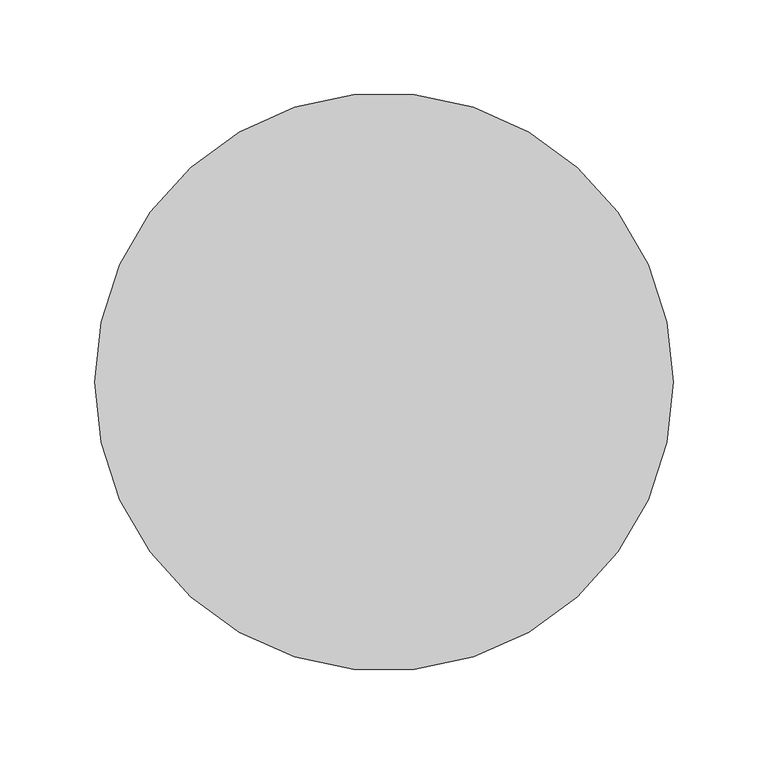
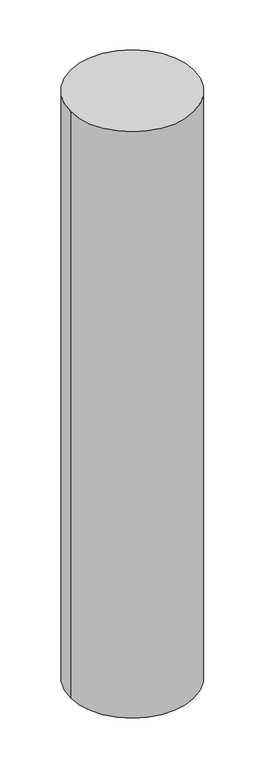
"""IFC4 building model written with IfcOpenShell, lengths in millimetres: proxy geometry."""

from ifc_helpers import new_model, si_unit, point, frame, frame_2d, origin, place, context, project, spatial, circle_curve, trimmed, segment, composite_curve, outline, extrude, source, transform, mapped, element, save


def generic_models_3ba2bbd2(model_context):
    return source(origin(), model_context, "Body", "SweptSolid", [
        extrude(outline(composite_curve([segment(trimmed(circle_curve(frame_2d((588972.4434739, -531724.9413841)), 152.4), [point((588820.0434739, -531724.9413841))], [point((589124.8434739, -531724.9413841))], False, "CARTESIAN"), True, "CONTINUOUS"), segment(trimmed(circle_curve(frame_2d((588972.4434739, -531724.9413841)), 152.4), [point((589124.8434739, -531724.9413841))], [point((588820.0434739, -531724.9413841))], False, "CARTESIAN"), True, "CONTINUOUS")], self_intersect=False)), frame((0.0, 0.0, -1676.4), z_axis=(0.0, 0.0, 1.0), x_axis=(1.0, 0.0, 0.0)), (0.0, 0.0, 1.0), 1524.0),
    ])


if __name__ == "__main__":
    model = new_model("IFC4")
    model_context = context("Model", 3, world=origin())
    ifc_project = project(units=[si_unit("LENGTHUNIT", "METRE", prefix="MILLI")], contexts=[model_context])
    site = spatial("IfcSite", under=ifc_project)
    building = spatial("IfcBuilding", under=site)
    placement = place(None, origin())
    generic_models_shape = generic_models_3ba2bbd2(model_context)
    element("IfcBuildingElementProxy", 1, Name="Sonotube Pier 1A : 12\" Sonotube Pier", ObjectType="Sonotube Pier 1A : 12\" Sonotube Pier", at=placement, inside=building, context=model_context, shape_type="MappedRepresentation", body=[
        mapped(generic_models_shape, transform((0.0, 0.0, 0.0), x_axis=(1.0, 0.0, 0.0), y_axis=(0.0, 1.0, 0.0), z_axis=(0.0, 0.0, 1.0))),
    ])
    save(model, "model.ifc")

# Revit data of these elements
# Element 1 (IfcBuildingElementProxy, "Sonotube Pier 1A : 12\" Sonotube Pier")
#   Materials on its faces: "12\" CONC SONOTUBE MIN. 60\" BELOW GRADE"
# Materials
#   "12\" CONC SONOTUBE MIN. 60\" BELOW GRADE": class "Generic", colour RGB 145 145 143, transparency 0, Cost = 0
